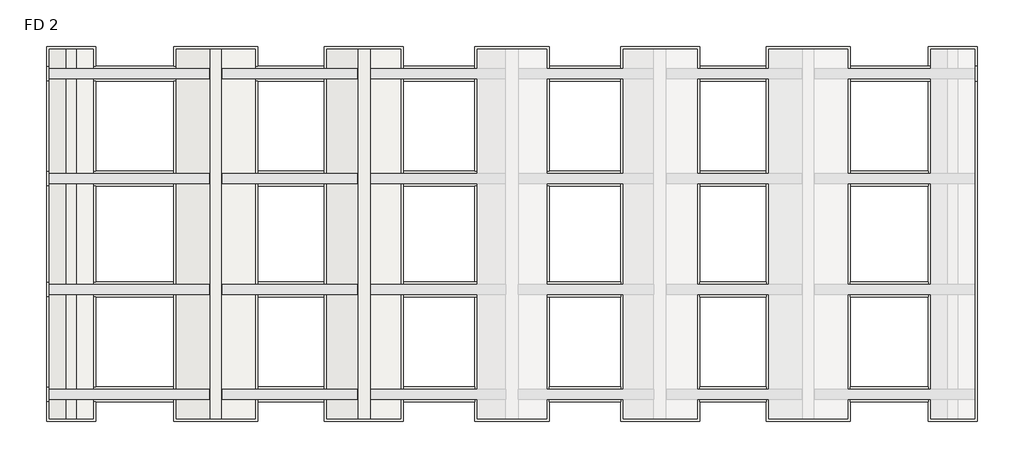
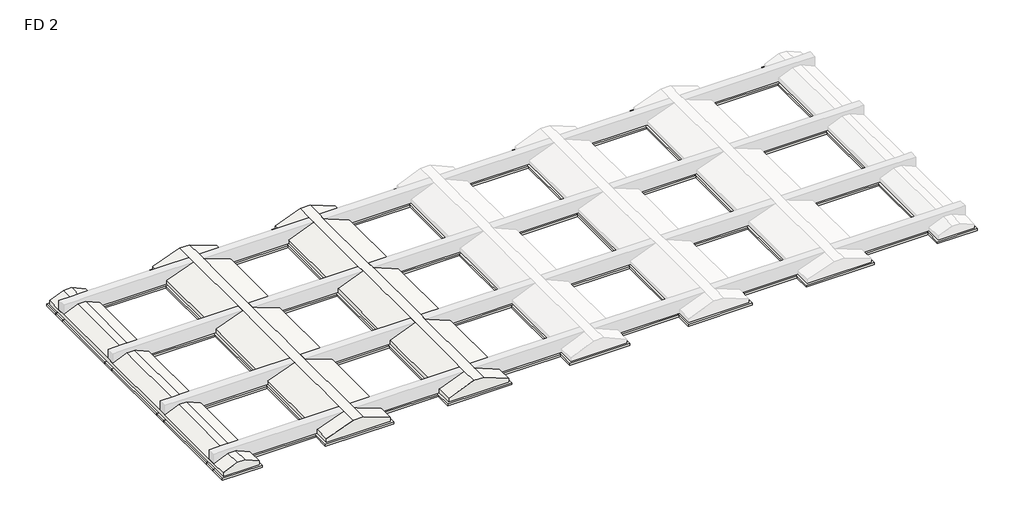
# One storey, part 1 of 2: 14 slabs.
"""IFC4 building model written with IfcOpenShell, lengths in millimetres."""

from ifc_helpers import new_model, si_unit, frame, origin, place, context, project, spatial, polyline, outline, extrude, faceted_brep, element, save

model = new_model("IFC4")

# Units and contexts
model_context = context("Model", 3, world=origin())
ifc_project = project(units=[si_unit("LENGTHUNIT", "METRE", prefix="MILLI")], contexts=[model_context])

# Site, building, storey
site = spatial("IfcSite", under=ifc_project)
building = spatial("IfcBuilding", under=site)
storey = spatial("IfcBuildingStorey", under=building, Name="FD 2", Elevation=-2170.0)

# Slabs
placement = place(None, origin())
element("IfcSlab", 1, ObjectType="Mong bang-lech tam : 1800x700", at=placement, inside=storey, context=model_context, shape_type="Brep", body=[
    faceted_brep([(-200.0, -999.9999998, -1670.0), (-900.0, -999.9999998, -1970.0), (-900.0, -999.9999998, -2170.0), (900.0, -999.9999998, -2170.0), (900.0, -999.9999998, -1970.0), (200.0, -999.9999998, -1670.0), (-200.0, 14000.0000002, -1670.0), (200.0, 14000.0000002, -1670.0), (900.0, 14000.0000002, -1970.0), (900.0, 14000.0000002, -2170.0), (-900.0, 14000.0000002, -2170.0), (-900.0, 14000.0000002, -1970.0), (-200.0, -200.0, -1670.0), (-200.0, 200.0, -1670.0), (-200.0, 4050.0000002, -1670.0), (-200.0, 4450.0000002, -1670.0), (-200.0, 8550.0000002, -1670.0), (-200.0, 8950.0000002, -1670.0), (-200.0, 12800.0000002, -1670.0), (-200.0, 13200.0000002, -1670.0), (-900.0, 13200.0000002, -1970.0), (-900.0, 12800.0000002, -1970.0), (-900.0, 8950.0000002, -1970.0), (-900.0, 8550.0000002, -1970.0), (-900.0, 4450.0000002, -1970.0), (-900.0, 4050.0000002, -1970.0), (-900.0, 200.0, -1970.0), (-900.0, -200.0, -1970.0), (900.0, 13200.0000002, -2170.0), (900.0, 12800.0000002, -2170.0), (900.0, 8950.0000002, -2170.0), (900.0, 8550.0000002, -2170.0), (900.0, 4450.0000002, -2170.0), (900.0, 4050.0000002, -2170.0), (900.0, 200.0, -2170.0), (900.0, -200.0, -2170.0), (900.0, 13200.0000002, -1970.0), (900.0, 12800.0000002, -1970.0), (900.0, 8950.0000002, -1970.0), (900.0, 8550.0000002, -1970.0), (900.0, 4450.0000002, -1970.0), (900.0, 4050.0000002, -1970.0), (900.0, 200.0, -1970.0), (900.0, -200.0, -1970.0), (200.0, 13200.0000002, -1670.0), (200.0, 12800.0000002, -1670.0), (200.0, 8950.0000002, -1670.0), (200.0, 8550.0000002, -1670.0), (200.0, 4450.0000002, -1670.0), (200.0, 4050.0000002, -1670.0), (200.0, 200.0, -1670.0), (200.0, -200.0, -1670.0)], [[[0, 1, 2, 3, 4, 5]], [[6, 7, 8, 9, 10, 11]], [[1, 0, 12, 13, 14, 15, 16, 17, 18, 19, 6, 11, 20, 21, 22, 23, 24, 25, 26, 27]], [[2, 1, 27, 26, 25, 24, 23, 22, 21, 20, 11, 10]], [[3, 2, 10, 9, 28, 29, 30, 31, 32, 33, 34, 35]], [[4, 3, 35, 34, 33, 32, 31, 30, 29, 28, 9, 8, 36, 37, 38, 39, 40, 41, 42, 43]], [[5, 4, 43, 42, 41, 40, 39, 38, 37, 36, 8, 7, 44, 45, 46, 47, 48, 49, 50, 51]], [[0, 5, 51, 50, 49, 48, 47, 46, 45, 44, 7, 6, 19, 18, 17, 16, 15, 14, 13, 12]]]),
])
element("IfcSlab", 2, ObjectType="2000x100", at=placement, inside=storey, context=model_context, shape_type="SweptSolid", body=[
    extrude(outline(polyline([(-1000.0, 14100.0000002), (1000.0, 14100.0000002), (1000.0, 13300.0000002), (-1000.0, 13300.0000002), (-1000.0, 14100.0000002)])), frame((0.0, 0.0, -2270.0), z_axis=(0.0, 0.0, 1.0), x_axis=(1.0, 0.0, 0.0)), (0.0, 0.0, 1.0), 100.0),
    extrude(outline(polyline([(1000.0, -1100.0), (-1000.0, -1100.0), (-1000.0, -300.0), (1000.0, -300.0), (1000.0, -1100.0)])), frame((0.0, 0.0, -2270.0), z_axis=(0.0, 0.0, 1.0), x_axis=(1.0, 0.0, 0.0)), (0.0, 0.0, 1.0), 100.0),
    extrude(outline(polyline([(-1000.0, 12700.0000002), (1000.0, 12700.0000002), (1000.0, 9050.0000002), (-1000.0, 9050.0000002), (-1000.0, 12700.0000002)])), frame((0.0, 0.0, -2270.0), z_axis=(0.0, 0.0, 1.0), x_axis=(1.0, 0.0, 0.0)), (0.0, 0.0, 1.0), 100.0),
    extrude(outline(polyline([(-1000.0, 8450.0000002), (1000.0, 8450.0000002), (1000.0, 4550.0000002), (-1000.0, 4550.0000002), (-1000.0, 8450.0000002)])), frame((0.0, 0.0, -2270.0), z_axis=(0.0, 0.0, 1.0), x_axis=(1.0, 0.0, 0.0)), (0.0, 0.0, 1.0), 100.0),
    extrude(outline(polyline([(-1000.0, 3950.0000002), (1000.0, 3950.0000002), (1000.0, 300.0), (-1000.0, 300.0), (-1000.0, 3950.0000002)])), frame((0.0, 0.0, -2270.0), z_axis=(0.0, 0.0, 1.0), x_axis=(1.0, 0.0, 0.0)), (0.0, 0.0, 1.0), 100.0),
])
element("IfcSlab", 3, ObjectType="2000x100", at=placement, inside=storey, context=model_context, shape_type="Brep", body=[
    faceted_brep([(34700.0350197, 14100.0000002, -2270.0), (36700.0350197, 14100.0000002, -2270.0), (36700.0350197, -1100.0, -2270.0), (34700.0350197, -1100.0, -2270.0), (34700.0350197, -300.0, -2270.0), (34700.0350197, 300.0, -2270.0), (34700.0350197, 3950.0000002, -2270.0), (34700.0350197, 4550.0000002, -2270.0), (34700.0350197, 8450.0000002, -2270.0), (34700.0350197, 9050.0000002, -2270.0), (34700.0350197, 12700.0000002, -2270.0), (36699.7667691, 12700.0000002, -2270.0), (36699.7667691, 13300.0000002, -2270.0), (34700.0350197, 13300.0000002, -2270.0), (36700.0350197, 14100.0000002, -2170.0), (34700.0350197, 14100.0000002, -2170.0), (34700.0350197, 13300.0000002, -2170.0), (36699.7667691, 13300.0000002, -2170.0), (36699.7667691, 12700.0000002, -2170.0), (34700.0350197, 12700.0000002, -2170.0), (34700.0350197, 9050.0000002, -2170.0), (34700.0350197, 8450.0000002, -2170.0), (34700.0350197, 4550.0000002, -2170.0), (34700.0350197, 3950.0000002, -2170.0), (34700.0350197, 300.0, -2170.0), (34700.0350197, -300.0, -2170.0), (34700.0350197, -1100.0, -2170.0), (36700.0350197, -1100.0, -2170.0)], [[[0, 1, 2, 3, 4, 5, 6, 7, 8, 9, 10, 11, 12, 13]], [[14, 15, 16, 17, 18, 19, 20, 21, 22, 23, 24, 25, 26, 27]], [[1, 0, 15, 14]], [[2, 1, 14, 27]], [[3, 2, 27, 26]], [[3, 26, 25, 24, 23, 22, 21, 20, 19, 10, 9, 8, 7, 6, 5, 4]], [[15, 0, 13, 16]], [[17, 12, 11, 18]], [[18, 11, 10, 19]], [[12, 17, 16, 13]]]),
])
element("IfcSlab", 4, ObjectType="3000x100", at=placement, inside=storey, context=model_context, shape_type="Brep", body=[
    faceted_brep([(16349.7667691, 14100.0000002, -2270.0), (19349.7667691, 14100.0000002, -2270.0), (19349.7667691, 13300.0000002, -2270.0), (19349.7667691, 12700.0000002, -2270.0), (19349.7667691, 9050.0000002, -2270.0), (16349.7667691, 9050.0000002, -2270.0), (16349.7667691, 12700.0000002, -2270.0), (16349.7667691, 13300.0000002, -2270.0), (19349.7667691, 14100.0000002, -2170.0), (16349.7667691, 14100.0000002, -2170.0), (16349.7667691, 13300.0000002, -2170.0), (16349.7667691, 12700.0000002, -2170.0), (16349.7667691, 9050.0000002, -2170.0), (19349.7667691, 9050.0000002, -2170.0), (19349.7667691, 12700.0000002, -2170.0), (19349.7667691, 13300.0000002, -2170.0)], [[[0, 1, 2, 3, 4, 5, 6, 7]], [[8, 9, 10, 11, 12, 13, 14, 15]], [[1, 0, 9, 8]], [[1, 8, 15, 14, 13, 4, 3, 2]], [[9, 0, 7, 6, 5, 12, 11, 10]], [[5, 4, 13, 12]]]),
    faceted_brep([(19349.7667691, -1100.0, -2270.0), (16349.7667691, -1100.0, -2270.0), (16349.7667691, -300.0, -2270.0), (16349.7667691, 300.0, -2270.0), (16349.7667691, 3950.0000002, -2270.0), (19349.7667691, 3950.0000002, -2270.0), (19349.7667691, 300.0, -2270.0), (19349.7667691, -300.0, -2270.0), (16349.7667691, -1100.0, -2170.0), (19349.7667691, -1100.0, -2170.0), (19349.7667691, -300.0, -2170.0), (19349.7667691, 300.0, -2170.0), (19349.7667691, 3950.0000002, -2170.0), (16349.7667691, 3950.0000002, -2170.0), (16349.7667691, 300.0, -2170.0), (16349.7667691, -300.0, -2170.0)], [[[0, 1, 2, 3, 4, 5, 6, 7]], [[8, 9, 10, 11, 12, 13, 14, 15]], [[9, 0, 7, 6, 5, 12, 11, 10]], [[1, 0, 9, 8]], [[1, 8, 15, 14, 13, 4, 3, 2]], [[5, 4, 13, 12]]]),
    faceted_brep([(19349.7667691, 4550.0000002, -2270.0), (16349.7667691, 4550.0000002, -2270.0), (16349.7667691, 8450.0000002, -2270.0), (19349.7667691, 8450.0000002, -2270.0), (16349.7667691, 4550.0000002, -2170.0), (19349.7667691, 4550.0000002, -2170.0), (19349.7667691, 8450.0000002, -2170.0), (16349.7667691, 8450.0000002, -2170.0)], [[[0, 1, 2, 3]], [[4, 5, 6, 7]], [[5, 0, 3, 6]], [[1, 4, 7, 2]], [[1, 0, 5, 4]], [[3, 2, 7, 6]]]),
])
element("IfcSlab", 5, ObjectType="Mong bang-lech tam : 3000x1000", at=placement, inside=storey, context=model_context, shape_type="Brep", body=[
    faceted_brep([(11599.9130239, -999.9999998, -1470.0), (10349.9130239, -999.9999998, -1970.0), (10349.9130239, -999.9999998, -2170.0), (13349.9130239, -999.9999998, -2170.0), (13349.9130239, -999.9999998, -1970.0), (12099.9130239, -999.9999998, -1470.0), (11599.9130239, 14000.0000002, -1470.0), (12099.9130239, 14000.0000002, -1470.0), (13349.9130239, 14000.0000002, -1970.0), (13349.9130239, 14000.0000002, -2170.0), (10349.9130239, 14000.0000002, -2170.0), (10349.9130239, 14000.0000002, -1970.0), (11599.9130239, -200.0, -1470.0), (11599.9130239, 200.0, -1470.0), (11599.9130239, 4050.0000002, -1470.0), (11599.9130239, 4450.0000002, -1470.0), (11599.9130239, 8550.0000002, -1470.0), (11599.9130239, 8950.0000002, -1470.0), (11599.9130239, 12800.0000002, -1470.0), (11599.9130239, 13200.0000002, -1470.0), (10349.9130239, 13200.0000002, -1970.0), (10349.9130239, 12800.0000002, -1970.0), (10349.9130239, 8950.0000002, -1970.0), (10349.9130239, 8550.0000002, -1970.0), (10349.9130239, 4450.0000002, -1970.0), (10349.9130239, 4050.0000002, -1970.0), (10349.9130239, 200.0, -1970.0), (10349.9130239, -200.0, -1970.0), (10349.9130239, 13200.0000002, -2170.0), (10349.9130239, 12800.0000002, -2170.0), (10349.9130239, 8950.0000002, -2170.0), (10349.9130239, 8550.0000002, -2170.0), (10349.9130239, 4450.0000002, -2170.0), (10349.9130239, 4050.0000002, -2170.0), (10349.9130239, 200.0, -2170.0), (10349.9130239, -200.0, -2170.0), (13349.9130239, 13200.0000002, -2170.0), (13349.9130239, 12800.0000002, -2170.0), (13349.9130239, 8950.0000002, -2170.0), (13349.9130239, 8550.0000002, -2170.0), (13349.9130239, 4450.0000002, -2170.0), (13349.9130239, 4050.0000002, -2170.0), (13349.9130239, 200.0, -2170.0), (13349.9130239, -200.0, -2170.0), (13349.9130239, 13200.0000002, -1970.0), (13349.9130239, 12800.0000002, -1970.0), (13349.9130239, 8950.0000002, -1970.0), (13349.9130239, 8550.0000002, -1970.0), (13349.9130239, 4450.0000002, -1970.0), (13349.9130239, 4050.0000002, -1970.0), (13349.9130239, 200.0, -1970.0), (13349.9130239, -200.0, -1970.0), (12099.9130239, 13200.0000002, -1470.0), (12099.9130239, 12800.0000002, -1470.0), (12099.9130239, 8950.0000002, -1470.0), (12099.9130239, 8550.0000002, -1470.0), (12099.9130239, 4450.0000002, -1470.0), (12099.9130239, 4050.0000002, -1470.0), (12099.9130239, 200.0, -1470.0), (12099.9130239, -200.0, -1470.0)], [[[0, 1, 2, 3, 4, 5]], [[6, 7, 8, 9, 10, 11]], [[1, 0, 12, 13, 14, 15, 16, 17, 18, 19, 6, 11, 20, 21, 22, 23, 24, 25, 26, 27]], [[2, 1, 27, 26, 25, 24, 23, 22, 21, 20, 11, 10, 28, 29, 30, 31, 32, 33, 34, 35]], [[3, 2, 35, 34, 33, 32, 31, 30, 29, 28, 10, 9, 36, 37, 38, 39, 40, 41, 42, 43]], [[4, 3, 43, 42, 41, 40, 39, 38, 37, 36, 9, 8, 44, 45, 46, 47, 48, 49, 50, 51]], [[5, 4, 51, 50, 49, 48, 47, 46, 45, 44, 8, 7, 52, 53, 54, 55, 56, 57, 58, 59]], [[0, 5, 59, 58, 57, 56, 55, 54, 53, 52, 7, 6, 19, 18, 17, 16, 15, 14, 13, 12]]]),
])
element("IfcSlab", 6, ObjectType="3200x100", at=placement, inside=storey, context=model_context, shape_type="Brep", body=[
    faceted_brep([(10250.0174941, 14100.0000002, -2270.0), (13450.0174941, 14100.0000002, -2270.0), (13450.0174941, 13300.0000002, -2270.0), (13450.0174941, 12700.0000002, -2270.0), (13450.0174941, 9050.0000002, -2270.0), (13450.0174941, 8450.0000002, -2270.0), (13450.0174941, 4550.0000002, -2270.0), (13450.0174941, 3950.0000002, -2270.0), (13450.0174941, 300.0, -2270.0), (13450.0174941, -300.0, -2270.0), (13450.0174941, -1100.0, -2270.0), (10250.0174941, -1100.0, -2270.0), (10250.0174941, -300.0, -2270.0), (10250.0174941, 300.0, -2270.0), (10250.0174941, 3950.0000002, -2270.0), (10250.0174941, 4550.0000002, -2270.0), (10250.0174941, 8450.0000002, -2270.0), (10250.0174941, 9050.0000002, -2270.0), (10250.0174941, 12700.0000002, -2270.0), (10250.0174941, 13300.0000002, -2270.0), (10250.0174941, 14100.0000002, -2170.0), (10250.0174941, 13300.0000002, -2170.0), (10250.0174941, 12700.0000002, -2170.0), (10250.0174941, 9050.0000002, -2170.0), (10250.0174941, 8450.0000002, -2170.0), (10250.0174941, 4550.0000002, -2170.0), (10250.0174941, 3950.0000002, -2170.0), (10250.0174941, 300.0, -2170.0), (10250.0174941, -300.0, -2170.0), (10250.0174941, -1100.0, -2170.0), (13450.0174941, -1100.0, -2170.0), (13450.0174941, -300.0, -2170.0), (13450.0174941, 300.0, -2170.0), (13450.0174941, 3950.0000002, -2170.0), (13450.0174941, 4550.0000002, -2170.0), (13450.0174941, 8450.0000002, -2170.0), (13450.0174941, 9050.0000002, -2170.0), (13450.0174941, 12700.0000002, -2170.0), (13450.0174941, 13300.0000002, -2170.0), (13450.0174941, 14100.0000002, -2170.0)], [[[0, 1, 2, 3, 4, 5, 6, 7, 8, 9, 10, 11, 12, 13, 14, 15, 16, 17, 18, 19]], [[20, 21, 22, 23, 24, 25, 26, 27, 28, 29, 30, 31, 32, 33, 34, 35, 36, 37, 38, 39]], [[1, 0, 20, 39]], [[10, 9, 8, 7, 6, 5, 4, 3, 2, 1, 39, 38, 37, 36, 35, 34, 33, 32, 31, 30]], [[11, 10, 30, 29]], [[0, 19, 18, 17, 16, 15, 14, 13, 12, 11, 29, 28, 27, 26, 25, 24, 23, 22, 21, 20]]]),
])
element("IfcSlab", 7, ObjectType="3200x100", at=placement, inside=storey, context=model_context, shape_type="Brep", body=[
    faceted_brep([(22250.0174954, 14100.0000002, -2270.0), (25450.0174954, 14100.0000002, -2270.0), (25450.0174954, 13300.0000002, -2270.0), (25450.0174954, 12700.0000002, -2270.0), (25450.0174954, 9050.0000002, -2270.0), (25450.0174954, 8450.0000002, -2270.0), (25450.0174954, 4550.0000002, -2270.0), (25450.0174954, 3950.0000002, -2270.0), (25450.0174954, 300.0, -2270.0), (25450.0174954, -300.0, -2270.0), (25450.0174954, -1100.0, -2270.0), (22250.0174954, -1100.0, -2270.0), (22250.0174954, -300.0, -2270.0), (22250.0174954, 300.0, -2270.0), (22250.0174954, 3950.0000002, -2270.0), (22250.0174954, 4550.0000002, -2270.0), (22250.0174954, 8450.0000002, -2270.0), (22250.0174954, 9050.0000002, -2270.0), (22250.0174954, 12700.0000002, -2270.0), (22250.0174954, 13300.0000002, -2270.0), (22250.0174954, 14100.0000002, -2170.0), (22250.0174954, 13300.0000002, -2170.0), (22250.0174954, 12700.0000002, -2170.0), (22250.0174954, 9050.0000002, -2170.0), (22250.0174954, 8450.0000002, -2170.0), (22250.0174954, 4550.0000002, -2170.0), (22250.0174954, 3950.0000002, -2170.0), (22250.0174954, 300.0, -2170.0), (22250.0174954, -300.0, -2170.0), (22250.0174954, -1100.0, -2170.0), (25450.0174954, -1100.0, -2170.0), (25450.0174954, -300.0, -2170.0), (25450.0174954, 300.0, -2170.0), (25450.0174954, 3950.0000002, -2170.0), (25450.0174954, 4550.0000002, -2170.0), (25450.0174954, 8450.0000002, -2170.0), (25450.0174954, 9050.0000002, -2170.0), (25450.0174954, 12700.0000002, -2170.0), (25450.0174954, 13300.0000002, -2170.0), (25450.0174954, 14100.0000002, -2170.0)], [[[0, 1, 2, 3, 4, 5, 6, 7, 8, 9, 10, 11, 12, 13, 14, 15, 16, 17, 18, 19]], [[20, 21, 22, 23, 24, 25, 26, 27, 28, 29, 30, 31, 32, 33, 34, 35, 36, 37, 38, 39]], [[1, 0, 20, 39]], [[10, 9, 8, 7, 6, 5, 4, 3, 2, 1, 39, 38, 37, 36, 35, 34, 33, 32, 31, 30]], [[11, 10, 30, 29]], [[0, 19, 18, 17, 16, 15, 14, 13, 12, 11, 29, 28, 27, 26, 25, 24, 23, 22, 21, 20]]]),
])
element("IfcSlab", 8, ObjectType="Mong bang-lech tam : 3200x1000", at=placement, inside=storey, context=model_context, shape_type="Brep", body=[
    faceted_brep([(5600.0000012, -999.9999998, -1470.0), (4250.0000012, -999.9999998, -1970.0), (4250.0000012, -999.9999998, -2170.0), (7450.0000012, -999.9999998, -2170.0), (7450.0000012, -999.9999998, -1970.0), (6100.0000012, -999.9999998, -1470.0), (7450.0000012, -200.0, -2170.0), (7450.0000012, 200.0, -2170.0), (7450.0000012, 4050.0000002, -2170.0), (7450.0000012, 4450.0000002, -2170.0), (7450.0000012, 8550.0000002, -2170.0), (7450.0000012, 8950.0000002, -2170.0), (7450.0000012, 12800.0000002, -2170.0), (7450.0000012, 13200.0000002, -2170.0), (7450.0000012, 14000.0000002, -2170.0), (7450.0000012, 14000.0000002, -1970.0), (7450.0000012, 13200.0000002, -1970.0), (7450.0000012, 12800.0000002, -1970.0), (7450.0000012, 8950.0000002, -1970.0), (7450.0000012, 8550.0000002, -1970.0), (7450.0000012, 4450.0000002, -1970.0), (7450.0000012, 4050.0000002, -1970.0), (7450.0000012, 200.0, -1970.0), (7450.0000012, -200.0, -1970.0), (6100.0000012, 14000.0000002, -1470.0), (6100.0000012, 13200.0000002, -1470.0), (6100.0000012, 12800.0000002, -1470.0), (6100.0000012, 8950.0000002, -1470.0), (6100.0000012, 8550.0000002, -1470.0), (6100.0000012, 4450.0000002, -1470.0), (6100.0000012, 4050.0000002, -1470.0), (6100.0000012, 200.0, -1470.0), (6100.0000012, -200.0, -1470.0), (5600.0000012, 14000.0000002, -1470.0), (5600.0000012, 13200.0000002, -1470.0), (5600.0000012, 12800.0000002, -1470.0), (5600.0000012, 8950.0000002, -1470.0), (5600.0000012, 8550.0000002, -1470.0), (5600.0000012, 4450.0000002, -1470.0), (5600.0000012, 4050.0000002, -1470.0), (5600.0000012, 200.0, -1470.0), (5600.0000012, -200.0, -1470.0), (4250.0000012, 14000.0000002, -2170.0), (4250.0000012, 14000.0000002, -1970.0), (4250.0000012, 13200.0000002, -1970.0), (4250.0000012, 12800.0000002, -1970.0), (4250.0000012, 8950.0000002, -1970.0), (4250.0000012, 8550.0000002, -1970.0), (4250.0000012, 4450.0000002, -1970.0), (4250.0000012, 4050.0000002, -1970.0), (4250.0000012, 200.0, -1970.0), (4250.0000012, -200.0, -1970.0), (4250.0000012, 13200.0000002, -2170.0), (4250.0000012, 12800.0000002, -2170.0), (4250.0000012, 8950.0000002, -2170.0), (4250.0000012, 8550.0000002, -2170.0), (4250.0000012, 4450.0000002, -2170.0), (4250.0000012, 4050.0000002, -2170.0), (4250.0000012, 200.0, -2170.0), (4250.0000012, -200.0, -2170.0)], [[[0, 1, 2, 3, 4, 5]], [[4, 3, 6, 7, 8, 9, 10, 11, 12, 13, 14, 15, 16, 17, 18, 19, 20, 21, 22, 23]], [[5, 4, 23, 22, 21, 20, 19, 18, 17, 16, 15, 24, 25, 26, 27, 28, 29, 30, 31, 32]], [[0, 5, 32, 31, 30, 29, 28, 27, 26, 25, 24, 33, 34, 35, 36, 37, 38, 39, 40, 41]], [[33, 24, 15, 14, 42, 43]], [[1, 0, 41, 40, 39, 38, 37, 36, 35, 34, 33, 43, 44, 45, 46, 47, 48, 49, 50, 51]], [[2, 1, 51, 50, 49, 48, 47, 46, 45, 44, 43, 42, 52, 53, 54, 55, 56, 57, 58, 59]], [[3, 2, 59, 58, 57, 56, 55, 54, 53, 52, 42, 14, 13, 12, 11, 10, 9, 8, 7, 6]]]),
])
element("IfcSlab", 9, ObjectType="3400x100", at=placement, inside=storey, context=model_context, shape_type="Brep", body=[
    faceted_brep([(4150.0000012, 14100.0000002, -2270.0), (7550.0000012, 14100.0000002, -2270.0), (7550.0000012, 13300.0000002, -2270.0), (4150.0000012, 13300.0000002, -2270.0), (7550.0000012, 14100.0000002, -2170.0), (4150.0000012, 14100.0000002, -2170.0), (4150.0000012, 13300.0000002, -2170.0), (7550.0000012, 13300.0000002, -2170.0)], [[[0, 1, 2, 3]], [[4, 5, 6, 7]], [[1, 0, 5, 4]], [[1, 4, 7, 2]], [[5, 0, 3, 6]], [[3, 2, 7, 6]]]),
    faceted_brep([(7550.0000012, -1100.0, -2270.0), (4150.0000012, -1100.0, -2270.0), (4150.0000012, -300.0, -2270.0), (4150.0000012, 300.0, -2270.0), (4150.0000012, 3950.0000002, -2270.0), (4150.0000012, 4550.0000002, -2270.0), (4150.0000012, 8450.0000002, -2270.0), (4150.0000012, 9050.0000002, -2270.0), (4150.0000012, 12700.0000002, -2270.0), (7550.0000012, 12700.0000002, -2270.0), (7550.0000012, 9050.0000002, -2270.0), (7550.0000012, 8450.0000002, -2270.0), (7550.0000012, 4550.0000002, -2270.0), (7550.0000012, 3950.0000002, -2270.0), (7550.0000012, 300.0, -2270.0), (7550.0000012, -300.0, -2270.0), (4150.0000012, -1100.0, -2170.0), (7550.0000012, -1100.0, -2170.0), (7550.0000012, -300.0, -2170.0), (7550.0000012, 300.0, -2170.0), (7550.0000012, 3950.0000002, -2170.0), (7550.0000012, 4550.0000002, -2170.0), (7550.0000012, 8450.0000002, -2170.0), (7550.0000012, 9050.0000002, -2170.0), (7550.0000012, 12700.0000002, -2170.0), (4150.0000012, 12700.0000002, -2170.0), (4150.0000012, 9050.0000002, -2170.0), (4150.0000012, 8450.0000002, -2170.0), (4150.0000012, 4550.0000002, -2170.0), (4150.0000012, 3950.0000002, -2170.0), (4150.0000012, 300.0, -2170.0), (4150.0000012, -300.0, -2170.0)], [[[0, 1, 2, 3, 4, 5, 6, 7, 8, 9, 10, 11, 12, 13, 14, 15]], [[16, 17, 18, 19, 20, 21, 22, 23, 24, 25, 26, 27, 28, 29, 30, 31]], [[17, 0, 15, 14, 13, 12, 11, 10, 9, 24, 23, 22, 21, 20, 19, 18]], [[1, 0, 17, 16]], [[1, 16, 31, 30, 29, 28, 27, 26, 25, 8, 7, 6, 5, 4, 3, 2]], [[9, 8, 25, 24]]]),
])
element("IfcSlab", 10, ObjectType="3400x100", at=placement, inside=storey, context=model_context, shape_type="Brep", body=[
    faceted_brep([(28150.0000043, 14100.0000002, -2270.0), (31550.0000043, 14100.0000002, -2270.0), (31550.0000043, 13300.0000002, -2270.0), (31550.0000043, 12700.0000002, -2270.0), (31550.0000043, 9050.0000002, -2270.0), (31550.0000043, 8450.0000002, -2270.0), (31550.0000043, 4550.0000002, -2270.0), (31550.0000043, 3950.0000002, -2270.0), (31550.0000043, 300.0, -2270.0), (31550.0000043, -300.0, -2270.0), (31550.0000043, -1100.0, -2270.0), (28150.0000043, -1100.0, -2270.0), (28150.0000043, -300.0, -2270.0), (28150.0000043, 300.0, -2270.0), (28150.0000043, 3950.0000002, -2270.0), (28150.0000043, 4550.0000002, -2270.0), (28150.0000043, 8450.0000002, -2270.0), (28150.0000043, 9050.0000002, -2270.0), (28150.0000043, 12700.0000002, -2270.0), (28150.0000043, 13300.0000002, -2270.0), (28150.0000043, 14100.0000002, -2170.0), (28150.0000043, 13300.0000002, -2170.0), (28150.0000043, 12700.0000002, -2170.0), (28150.0000043, 9050.0000002, -2170.0), (28150.0000043, 8450.0000002, -2170.0), (28150.0000043, 4550.0000002, -2170.0), (28150.0000043, 3950.0000002, -2170.0), (28150.0000043, 300.0, -2170.0), (28150.0000043, -300.0, -2170.0), (28150.0000043, -1100.0, -2170.0), (31550.0000043, -1100.0, -2170.0), (31550.0000043, -300.0, -2170.0), (31550.0000043, 300.0, -2170.0), (31550.0000043, 3950.0000002, -2170.0), (31550.0000043, 4550.0000002, -2170.0), (31550.0000043, 8450.0000002, -2170.0), (31550.0000043, 9050.0000002, -2170.0), (31550.0000043, 12700.0000002, -2170.0), (31550.0000043, 13300.0000002, -2170.0), (31550.0000043, 14100.0000002, -2170.0)], [[[0, 1, 2, 3, 4, 5, 6, 7, 8, 9, 10, 11, 12, 13, 14, 15, 16, 17, 18, 19]], [[20, 21, 22, 23, 24, 25, 26, 27, 28, 29, 30, 31, 32, 33, 34, 35, 36, 37, 38, 39]], [[1, 0, 20, 39]], [[10, 9, 8, 7, 6, 5, 4, 3, 2, 1, 39, 38, 37, 36, 35, 34, 33, 32, 31, 30]], [[11, 10, 30, 29]], [[0, 19, 18, 17, 16, 15, 14, 13, 12, 11, 29, 28, 27, 26, 25, 24, 23, 22, 21, 20]]]),
])
element("IfcSlab", 11, ObjectType="600x100", at=placement, inside=storey, context=model_context, shape_type="Brep", body=[
    faceted_brep([(-1000.0, 12700.0000002, -2270.0), (-1000.0, 13300.0000002, -2270.0), (1000.0, 13300.0000002, -2270.0), (4150.0000012, 13300.0000002, -2270.0), (7550.0000012, 13300.0000002, -2270.0), (10250.0174941, 13300.0000002, -2270.0), (10250.0174941, 12700.0000002, -2270.0), (7550.0000012, 12700.0000002, -2270.0), (4150.0000012, 12700.0000002, -2270.0), (1000.0, 12700.0000002, -2270.0), (-1000.0, 13300.0000002, -2170.0), (-1000.0, 12700.0000002, -2170.0), (1000.0, 12700.0000002, -2170.0), (4150.0000012, 12700.0000002, -2170.0), (7550.0000012, 12700.0000002, -2170.0), (10250.0174941, 12700.0000002, -2170.0), (10250.0174941, 13300.0000002, -2170.0), (7550.0000012, 13300.0000002, -2170.0), (4150.0000012, 13300.0000002, -2170.0), (1000.0, 13300.0000002, -2170.0)], [[[0, 1, 2, 3, 4, 5, 6, 7, 8, 9]], [[10, 11, 12, 13, 14, 15, 16, 17, 18, 19]], [[11, 0, 9, 8, 7, 6, 15, 14, 13, 12]], [[1, 0, 11, 10]], [[1, 10, 19, 18, 17, 16, 5, 4, 3, 2]], [[6, 5, 16, 15]]]),
    faceted_brep([(19349.7667691, 12700.0000002, -2270.0), (19349.7667691, 13300.0000002, -2270.0), (22250.0174954, 13300.0000002, -2270.0), (22250.0174954, 12700.0000002, -2270.0), (19349.7667691, 13300.0000002, -2170.0), (19349.7667691, 12700.0000002, -2170.0), (22250.0174954, 12700.0000002, -2170.0), (22250.0174954, 13300.0000002, -2170.0)], [[[0, 1, 2, 3]], [[4, 5, 6, 7]], [[5, 0, 3, 6]], [[1, 0, 5, 4]], [[1, 4, 7, 2]], [[3, 2, 7, 6]]]),
    faceted_brep([(16349.7667691, 13300.0000002, -2270.0), (16349.7667691, 12700.0000002, -2270.0), (13450.0174941, 12700.0000002, -2270.0), (13450.0174941, 13300.0000002, -2270.0), (16349.7667691, 12700.0000002, -2170.0), (16349.7667691, 13300.0000002, -2170.0), (13450.0174941, 13300.0000002, -2170.0), (13450.0174941, 12700.0000002, -2170.0)], [[[0, 1, 2, 3]], [[4, 5, 6, 7]], [[1, 4, 7, 2]], [[1, 0, 5, 4]], [[5, 0, 3, 6]], [[3, 2, 7, 6]]]),
    faceted_brep([(25450.0174954, 12700.0000002, -2270.0), (25450.0174954, 13300.0000002, -2270.0), (28150.0000043, 13300.0000002, -2270.0), (28150.0000043, 12700.0000002, -2270.0), (25450.0174954, 13300.0000002, -2170.0), (25450.0174954, 12700.0000002, -2170.0), (28150.0000043, 12700.0000002, -2170.0), (28150.0000043, 13300.0000002, -2170.0)], [[[0, 1, 2, 3]], [[4, 5, 6, 7]], [[5, 0, 3, 6]], [[1, 4, 7, 2]], [[1, 0, 5, 4]], [[3, 2, 7, 6]]]),
    faceted_brep([(36699.7667691, 13300.0000002, -2270.0), (36699.7667691, 12700.0000002, -2270.0), (34700.0350197, 12700.0000002, -2270.0), (31550.0000043, 12700.0000002, -2270.0), (31550.0000043, 13300.0000002, -2270.0), (34700.0350197, 13300.0000002, -2270.0), (36699.7667691, 12700.0000002, -2170.0), (36699.7667691, 13300.0000002, -2170.0), (34700.0350197, 13300.0000002, -2170.0), (31550.0000043, 13300.0000002, -2170.0), (31550.0000043, 12700.0000002, -2170.0), (34700.0350197, 12700.0000002, -2170.0)], [[[0, 1, 2, 3, 4, 5]], [[6, 7, 8, 9, 10, 11]], [[1, 0, 7, 6]], [[1, 6, 11, 10, 3, 2]], [[7, 0, 5, 4, 9, 8]], [[4, 3, 10, 9]]]),
])
element("IfcSlab", 12, ObjectType="600x100", at=placement, inside=storey, context=model_context, shape_type="Brep", body=[
    faceted_brep([(-1000.0, 8450.0000002, -2270.0), (-1000.0, 9050.0000002, -2270.0), (1000.0, 9050.0000002, -2270.0), (4150.0000012, 9050.0000002, -2270.0), (4150.0000012, 8450.0000002, -2270.0), (1000.0, 8450.0000002, -2270.0), (-1000.0, 9050.0000002, -2170.0), (-1000.0, 8450.0000002, -2170.0), (1000.0, 8450.0000002, -2170.0), (4150.0000012, 8450.0000002, -2170.0), (4150.0000012, 9050.0000002, -2170.0), (1000.0, 9050.0000002, -2170.0)], [[[0, 1, 2, 3, 4, 5]], [[6, 7, 8, 9, 10, 11]], [[7, 0, 5, 4, 9, 8]], [[1, 0, 7, 6]], [[1, 6, 11, 10, 3, 2]], [[4, 3, 10, 9]]]),
    faceted_brep([(7550.0000012, 8450.0000002, -2270.0), (7550.0000012, 9050.0000002, -2270.0), (10250.0174941, 9050.0000002, -2270.0), (10250.0174941, 8450.0000002, -2270.0), (7550.0000012, 9050.0000002, -2170.0), (7550.0000012, 8450.0000002, -2170.0), (10250.0174941, 8450.0000002, -2170.0), (10250.0174941, 9050.0000002, -2170.0)], [[[0, 1, 2, 3]], [[4, 5, 6, 7]], [[5, 0, 3, 6]], [[1, 4, 7, 2]], [[1, 0, 5, 4]], [[3, 2, 7, 6]]]),
    faceted_brep([(13450.0174941, 8450.0000002, -2270.0), (13450.0174941, 9050.0000002, -2270.0), (16349.7667691, 9050.0000002, -2270.0), (19349.7667691, 9050.0000002, -2270.0), (22250.0174954, 9050.0000002, -2270.0), (22250.0174954, 8450.0000002, -2270.0), (19349.7667691, 8450.0000002, -2270.0), (16349.7667691, 8450.0000002, -2270.0), (13450.0174941, 9050.0000002, -2170.0), (13450.0174941, 8450.0000002, -2170.0), (16349.7667691, 8450.0000002, -2170.0), (19349.7667691, 8450.0000002, -2170.0), (22250.0174954, 8450.0000002, -2170.0), (22250.0174954, 9050.0000002, -2170.0), (19349.7667691, 9050.0000002, -2170.0), (16349.7667691, 9050.0000002, -2170.0)], [[[0, 1, 2, 3, 4, 5, 6, 7]], [[8, 9, 10, 11, 12, 13, 14, 15]], [[9, 0, 7, 6, 5, 12, 11, 10]], [[1, 8, 15, 14, 13, 4, 3, 2]], [[1, 0, 9, 8]], [[5, 4, 13, 12]]]),
    faceted_brep([(25450.0174954, 8450.0000002, -2270.0), (25450.0174954, 9050.0000002, -2270.0), (28150.0000043, 9050.0000002, -2270.0), (28150.0000043, 8450.0000002, -2270.0), (25450.0174954, 9050.0000002, -2170.0), (25450.0174954, 8450.0000002, -2170.0), (28150.0000043, 8450.0000002, -2170.0), (28150.0000043, 9050.0000002, -2170.0)], [[[0, 1, 2, 3]], [[4, 5, 6, 7]], [[5, 0, 3, 6]], [[1, 4, 7, 2]], [[1, 0, 5, 4]], [[3, 2, 7, 6]]]),
    faceted_brep([(31550.0000043, 8450.0000002, -2270.0), (31550.0000043, 9050.0000002, -2270.0), (34700.0350197, 9050.0000002, -2270.0), (34700.0350197, 8450.0000002, -2270.0), (31550.0000043, 9050.0000002, -2170.0), (31550.0000043, 8450.0000002, -2170.0), (34700.0350197, 8450.0000002, -2170.0), (34700.0350197, 9050.0000002, -2170.0)], [[[0, 1, 2, 3]], [[4, 5, 6, 7]], [[5, 0, 3, 6]], [[1, 4, 7, 2]], [[1, 0, 5, 4]], [[3, 2, 7, 6]]]),
])
element("IfcSlab", 13, ObjectType="600x100", at=placement, inside=storey, context=model_context, shape_type="Brep", body=[
    faceted_brep([(-1000.0, 3950.0000002, -2270.0), (-1000.0, 4550.0000002, -2270.0), (1000.0, 4550.0000002, -2270.0), (4150.0000012, 4550.0000002, -2270.0), (4150.0000012, 3950.0000002, -2270.0), (1000.0, 3950.0000002, -2270.0), (-1000.0, 4550.0000002, -2170.0), (-1000.0, 3950.0000002, -2170.0), (1000.0, 3950.0000002, -2170.0), (4150.0000012, 3950.0000002, -2170.0), (4150.0000012, 4550.0000002, -2170.0), (1000.0, 4550.0000002, -2170.0)], [[[0, 1, 2, 3, 4, 5]], [[6, 7, 8, 9, 10, 11]], [[7, 0, 5, 4, 9, 8]], [[1, 0, 7, 6]], [[1, 6, 11, 10, 3, 2]], [[4, 3, 10, 9]]]),
    faceted_brep([(7550.0000012, 3950.0000002, -2270.0), (7550.0000012, 4550.0000002, -2270.0), (10250.0174941, 4550.0000002, -2270.0), (10250.0174941, 3950.0000002, -2270.0), (7550.0000012, 4550.0000002, -2170.0), (7550.0000012, 3950.0000002, -2170.0), (10250.0174941, 3950.0000002, -2170.0), (10250.0174941, 4550.0000002, -2170.0)], [[[0, 1, 2, 3]], [[4, 5, 6, 7]], [[5, 0, 3, 6]], [[1, 4, 7, 2]], [[1, 0, 5, 4]], [[3, 2, 7, 6]]]),
    faceted_brep([(13450.0174941, 3950.0000002, -2270.0), (13450.0174941, 4550.0000002, -2270.0), (16349.7667691, 4550.0000002, -2270.0), (19349.7667691, 4550.0000002, -2270.0), (22250.0174954, 4550.0000002, -2270.0), (22250.0174954, 3950.0000002, -2270.0), (19349.7667691, 3950.0000002, -2270.0), (16349.7667691, 3950.0000002, -2270.0), (13450.0174941, 4550.0000002, -2170.0), (13450.0174941, 3950.0000002, -2170.0), (16349.7667691, 3950.0000002, -2170.0), (19349.7667691, 3950.0000002, -2170.0), (22250.0174954, 3950.0000002, -2170.0), (22250.0174954, 4550.0000002, -2170.0), (19349.7667691, 4550.0000002, -2170.0), (16349.7667691, 4550.0000002, -2170.0)], [[[0, 1, 2, 3, 4, 5, 6, 7]], [[8, 9, 10, 11, 12, 13, 14, 15]], [[9, 0, 7, 6, 5, 12, 11, 10]], [[1, 8, 15, 14, 13, 4, 3, 2]], [[1, 0, 9, 8]], [[5, 4, 13, 12]]]),
    faceted_brep([(25450.0174954, 3950.0000002, -2270.0), (25450.0174954, 4550.0000002, -2270.0), (28150.0000043, 4550.0000002, -2270.0), (28150.0000043, 3950.0000002, -2270.0), (25450.0174954, 4550.0000002, -2170.0), (25450.0174954, 3950.0000002, -2170.0), (28150.0000043, 3950.0000002, -2170.0), (28150.0000043, 4550.0000002, -2170.0)], [[[0, 1, 2, 3]], [[4, 5, 6, 7]], [[5, 0, 3, 6]], [[1, 4, 7, 2]], [[1, 0, 5, 4]], [[3, 2, 7, 6]]]),
    faceted_brep([(31550.0000043, 3950.0000002, -2270.0), (31550.0000043, 4550.0000002, -2270.0), (34700.0350197, 4550.0000002, -2270.0), (34700.0350197, 3950.0000002, -2270.0), (31550.0000043, 4550.0000002, -2170.0), (31550.0000043, 3950.0000002, -2170.0), (34700.0350197, 3950.0000002, -2170.0), (34700.0350197, 4550.0000002, -2170.0)], [[[0, 1, 2, 3]], [[4, 5, 6, 7]], [[5, 0, 3, 6]], [[1, 4, 7, 2]], [[1, 0, 5, 4]], [[3, 2, 7, 6]]]),
])
element("IfcSlab", 14, ObjectType="600x100", at=placement, inside=storey, context=model_context, shape_type="Brep", body=[
    faceted_brep([(-1000.0, -300.0, -2270.0), (-1000.0, 300.0, -2270.0), (1000.0, 300.0, -2270.0), (4150.0000012, 300.0, -2270.0), (4150.0000012, -300.0, -2270.0), (1000.0, -300.0, -2270.0), (-1000.0, 300.0, -2170.0), (-1000.0, -300.0, -2170.0), (1000.0, -300.0, -2170.0), (4150.0000012, -300.0, -2170.0), (4150.0000012, 300.0, -2170.0), (1000.0, 300.0, -2170.0)], [[[0, 1, 2, 3, 4, 5]], [[6, 7, 8, 9, 10, 11]], [[7, 0, 5, 4, 9, 8]], [[1, 0, 7, 6]], [[1, 6, 11, 10, 3, 2]], [[4, 3, 10, 9]]]),
    faceted_brep([(13450.0174941, -300.0, -2270.0), (13450.0174941, 300.0, -2270.0), (16349.7667691, 300.0, -2270.0), (16349.7667691, -300.0, -2270.0), (13450.0174941, 300.0, -2170.0), (13450.0174941, -300.0, -2170.0), (16349.7667691, -300.0, -2170.0), (16349.7667691, 300.0, -2170.0)], [[[0, 1, 2, 3]], [[4, 5, 6, 7]], [[5, 0, 3, 6]], [[1, 4, 7, 2]], [[1, 0, 5, 4]], [[3, 2, 7, 6]]]),
    faceted_brep([(10250.0174941, 300.0, -2270.0), (10250.0174941, -300.0, -2270.0), (7550.0000012, -300.0, -2270.0), (7550.0000012, 300.0, -2270.0), (10250.0174941, -300.0, -2170.0), (10250.0174941, 300.0, -2170.0), (7550.0000012, 300.0, -2170.0), (7550.0000012, -300.0, -2170.0)], [[[0, 1, 2, 3]], [[4, 5, 6, 7]], [[1, 4, 7, 2]], [[5, 0, 3, 6]], [[1, 0, 5, 4]], [[3, 2, 7, 6]]]),
    faceted_brep([(19349.7667691, -300.0, -2270.0), (19349.7667691, 300.0, -2270.0), (22250.0174954, 300.0, -2270.0), (22250.0174954, -300.0, -2270.0), (19349.7667691, 300.0, -2170.0), (19349.7667691, -300.0, -2170.0), (22250.0174954, -300.0, -2170.0), (22250.0174954, 300.0, -2170.0)], [[[0, 1, 2, 3]], [[4, 5, 6, 7]], [[5, 0, 3, 6]], [[1, 4, 7, 2]], [[1, 0, 5, 4]], [[3, 2, 7, 6]]]),
    faceted_brep([(25450.0174954, -300.0, -2270.0), (25450.0174954, 300.0, -2270.0), (28150.0000043, 300.0, -2270.0), (28150.0000043, -300.0, -2270.0), (25450.0174954, 300.0, -2170.0), (25450.0174954, -300.0, -2170.0), (28150.0000043, -300.0, -2170.0), (28150.0000043, 300.0, -2170.0)], [[[0, 1, 2, 3]], [[4, 5, 6, 7]], [[5, 0, 3, 6]], [[1, 4, 7, 2]], [[1, 0, 5, 4]], [[3, 2, 7, 6]]]),
    faceted_brep([(31550.0000043, -300.0, -2270.0), (31550.0000043, 300.0, -2270.0), (34700.0350197, 300.0, -2270.0), (34700.0350197, -300.0, -2270.0), (31550.0000043, 300.0, -2170.0), (31550.0000043, -300.0, -2170.0), (34700.0350197, -300.0, -2170.0), (34700.0350197, 300.0, -2170.0)], [[[0, 1, 2, 3]], [[4, 5, 6, 7]], [[5, 0, 3, 6]], [[1, 4, 7, 2]], [[1, 0, 5, 4]], [[3, 2, 7, 6]]]),
])

save(model, "model.ifc")

# Revit data of these elements
# Project information
#   Project Issue Date = "29/09/2021"
#   Project Status = "FC DWR 29/07/2021"
#   Client Name = "Owner"
#   Project Address = "LOT TT1, Tan Phu Trung Industrial Park,\n Tan Phu Trung Town, Cu Chi District, Ho Chi Minh, Viet Nam"
#   Project Name = "DỰ ÁN 27"
#   Project Number = "0001"
#   SR Document GUID = "5b4f20b2-f425-4572-8575-adb942fb322d"
# Grids (mm)
#   "B": line (39750.018, 4350) -> (-2567.1, 4350)
#   "3": line (11850, -4100.379) -> (11850, 16640.319)
#   "4": line (17850, -4100.379) -> (17850, 16640.319)
#   "5": line (23850, -4100.379) -> (23850, 16640.319)
#   "2": line (5850, -4100.379) -> (5850, 16640.319)
#   "7": line (35700.035, -4100.379) -> (35700.035, 16640.319)
#   "1": line (0, -4100.379) -> (0, 16640.319)
#   "A": line (39750.018, 0) -> (-2567.1, 0)
#   "C": line (39750.018, 8650) -> (-2567.1, 8650)
#   "D": line (39750.018, 13000) -> (-2567.1, 13000)
#   "6": line (29850, -4100.379) -> (29850, 16640.319)
# Type "Mong bang-lech tam : 1800x700"
#   Length = 15000 mm
#   Lech Tam (E) = 0 mm
#   Foundation Thickness = 500 mm
#   Foundation (h2) = 200 mm
#   Foundation (h1) = 300 mm
#   Be Rong Dam (b) = 400 mm
#   Be Rong Dai Mong (B) = 1800 mm
#   Structural Material [instance default] = Concrete, Cast-in-Place gray
#   Width = 0
#   Assembly Code = ""
# Type "2000x100"
#   Function = 0
#   Layers, outside or top first: 100 mm "VM.TM1A-Concrete Wall-M250" (function 1)
# Type "3000x100"
#   Function = 0
#   Layers, outside or top first: 100 mm "VM.TM1A-Concrete Wall-M250" (function 1)
# Type "Mong bang-lech tam : 3000x1000"
#   Length = 15000 mm
#   Lech Tam (E) = 0 mm
#   Foundation Thickness = 700 mm
#   Foundation (h2) = 200 mm
#   Foundation (h1) = 500 mm
#   Be Rong Dam (b) = 500 mm
#   Be Rong Dai Mong (B) = 3000 mm
#   Structural Material [instance default] = Concrete, Cast-in-Place gray
#   Width = 0
#   Assembly Code = ""
# Type "3200x100"
#   Function = 0
#   Layers, outside or top first: 100 mm "VM.TM1A-Concrete Wall-M250" (function 1)
# Type "Mong bang-lech tam : 3200x1000"
#   Length = 15000 mm
#   Lech Tam (E) = 0 mm
#   Foundation Thickness = 700 mm
#   Foundation (h2) = 200 mm
#   Foundation (h1) = 500 mm
#   Be Rong Dam (b) = 500 mm
#   Be Rong Dai Mong (B) = 3200 mm
#   Structural Material [instance default] = Concrete, Cast-in-Place gray
#   Width = 0
#   Assembly Code = ""
# Type "3400x100"
#   Function = 0
#   Layers, outside or top first: 100 mm "VM.TM1A-Concrete Wall-M250" (function 1)
# Type "600x100"
#   Function = 0
#   Layers, outside or top first: 100 mm "VM.TM1A-Concrete Wall-M250" (function 1)
# Element 1 (IfcSlab, "Mong bang-lech tam : 1800x700")
#   COF_CON__WorkItemNumber = "SH3-A-GF"
#   COF_GEN__Name = "MB4"
#   Structural Material = Concrete, Cast-in-Place gray
#   Phase Created = New Construction
#   Materials on its faces: "Concrete, Cast-in-Place gray"
# Elements 2, 3 (IfcSlab, "2000x100")
#   COF_CON__WorkItemNumber = "SH3-A-GF"
#   COF_GEN__Name = "BTLM"
#   built-in parameter 1001955 = 3.14159 (stored number, unit not read)
#   Height Offset From Level = 0 mm
#   Phase Created = New Construction
#   Materials on its faces: "VM.TM1A-Concrete Wall-M250"
# Element 4 (IfcSlab, "3000x100")
#   COF_CON__WorkItemNumber = "SH3-A-GF"
#   COF_GEN__Name = "BTLM"
#   built-in parameter 1001955 = 3.14159 (stored number, unit not read)
#   Height Offset From Level = 0 mm
#   Phase Created = New Construction
#   Materials on its faces: "VM.TM1A-Concrete Wall-M250"
# Element 5 (IfcSlab, "Mong bang-lech tam : 3000x1000")
#   COF_CON__WorkItemNumber = "SH3-A-GF"
#   COF_GEN__Name = "MB2"
#   Structural Material = Concrete, Cast-in-Place gray
#   Phase Created = New Construction
#   Materials on its faces: "Concrete, Cast-in-Place gray"
# Elements 6, 7 (IfcSlab, "3200x100")
#   COF_CON__WorkItemNumber = "SH3-A-GF"
#   COF_GEN__Name = "BTLM"
#   built-in parameter 1001955 = 3.14159 (stored number, unit not read)
#   Height Offset From Level = 0 mm
#   Phase Created = New Construction
#   Materials on its faces: "VM.TM1A-Concrete Wall-M250"
# Element 8 (IfcSlab, "Mong bang-lech tam : 3200x1000")
#   COF_CON__WorkItemNumber = "SH3-A-GF"
#   COF_GEN__Name = "MB1"
#   Structural Material = Concrete, Cast-in-Place gray
#   Phase Created = New Construction
#   Materials on its faces: "Concrete, Cast-in-Place gray"
# Elements 9, 10 (IfcSlab, "3400x100")
#   COF_CON__WorkItemNumber = "SH3-A-GF"
#   COF_GEN__Name = "BTLM"
#   built-in parameter 1001955 = 3.14159 (stored number, unit not read)
#   Height Offset From Level = 0 mm
#   Phase Created = New Construction
#   Materials on its faces: "VM.TM1A-Concrete Wall-M250"
# Elements 11, 12, 13, 14 (IfcSlab, "600x100")
#   COF_CON__WorkItemNumber = "SH3-A-GF"
#   COF_GEN__Name = "BTLM"
#   Height Offset From Level = 0 mm
#   Phase Created = New Construction
#   Materials on its faces: "VM.TM1A-Concrete Wall-M250"
# Materials
#   "Concrete, Cast-in-Place gray": class "Concrete", colour RGB 207 208 204, transparency 0, Description = "Cast-in-place concrete", Cost = 0
#   "VM.TM1A-Concrete Wall-M250": class "Concrete", colour RGB 192 192 192, transparency 0, Description = "Cast-in-place concrete", Cost = 0
